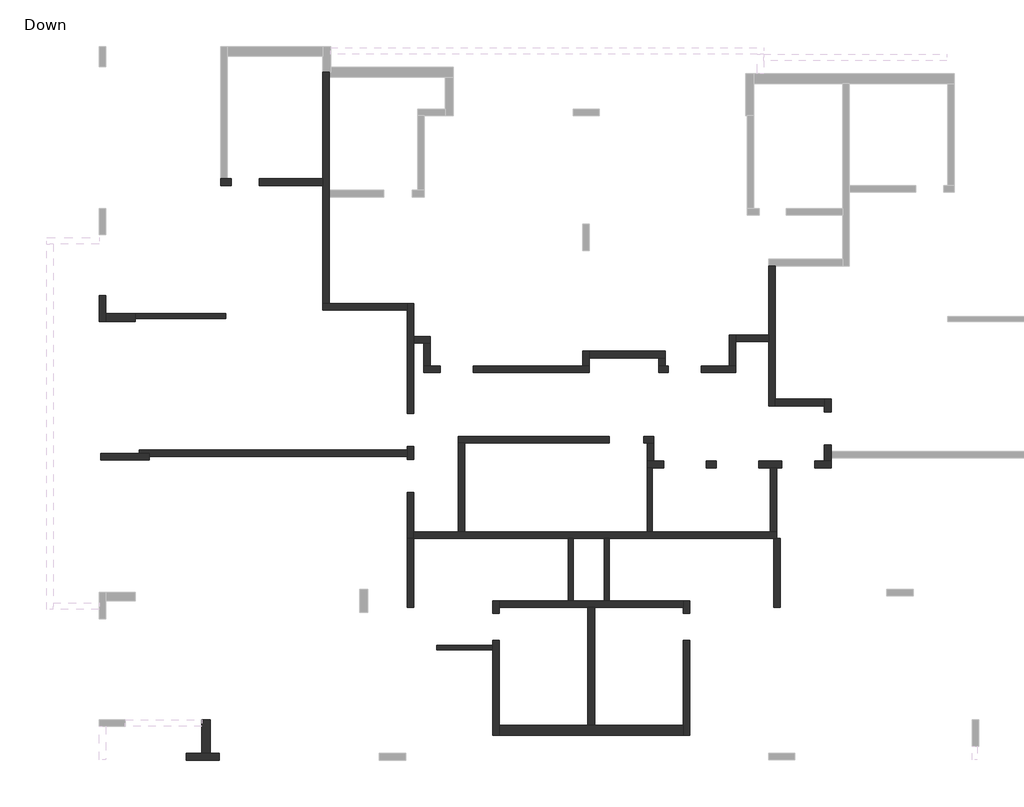
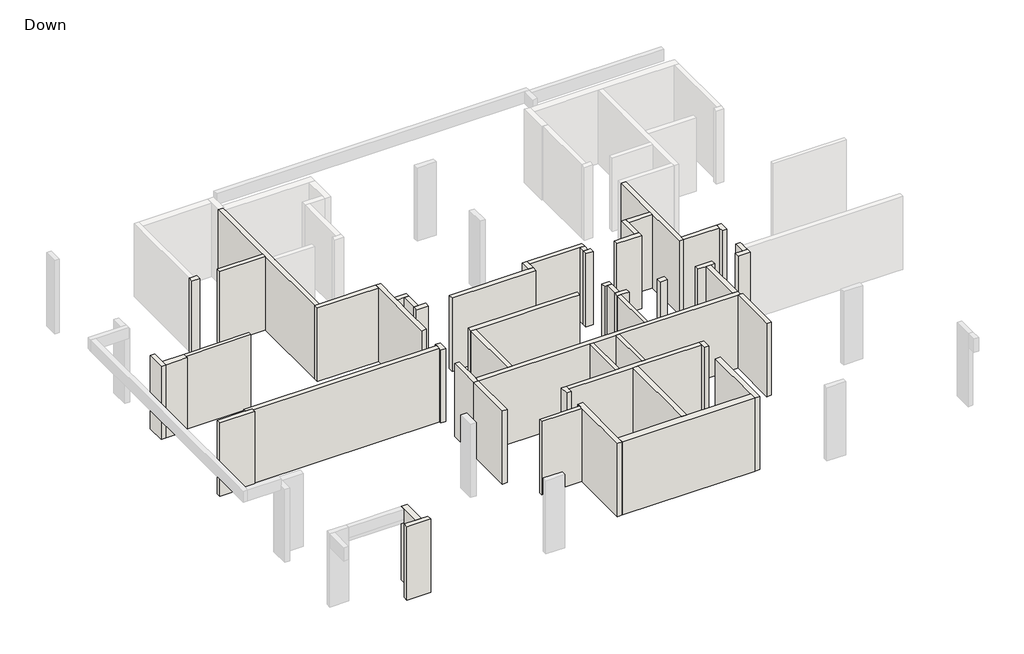
# One storey, part 1 of 2: 52 walls.
"""IFC4 building model written with IfcOpenShell, lengths in millimetres."""

import ifcopenshell
import ifcopenshell.guid

model = None  # the IFC model being written
_history = None  # IfcOwnerHistory: only IFC2X3 demands one
_inside = {}  # id of a spatial element -> (the spatial element, [elements in it])
_under = {}  # id of a project, library or spatial element -> (it, [spatial elements below it])
_declared = {}  # id of a project -> (the project, [libraries it declares])
_typed = {}  # id of a type object -> (the type object, [elements of that type])
_made_of = {}  # id of a material, layer set ... -> (it, [elements and type objects made of it])


def new_model(schema):
    """Start an empty IFC model of exactly this schema.

    Asked for "IFC4X3", IfcOpenShell would pick the latest addendum, in which some entities
    have other attributes; the version numbers below select the first issue.
    IFC2X3 requires an IfcOwnerHistory on every rooted entity: one is made here for all.
    """
    global model, _history
    if schema == "IFC4X3":
        model = ifcopenshell.file(schema_version=(4, 3, 0, 0))
    else:
        model = ifcopenshell.file(schema=schema)
    _inside.clear()
    _under.clear()
    _declared.clear()
    _typed.clear()
    _made_of.clear()
    _history = None
    if model.schema == "IFC2X3":
        org = make("IfcOrganization", Name="unknown")
        user = make(
            "IfcPersonAndOrganization",
            ThePerson=make("IfcPerson", FamilyName="unknown"),
            TheOrganization=org,
        )
        app = make(
            "IfcApplication",
            ApplicationDeveloper=org,
            Version="unknown",
            ApplicationFullName="unknown",
            ApplicationIdentifier="unknown",
        )
        _history = make(
            "IfcOwnerHistory",
            OwningUser=user,
            OwningApplication=app,
            ChangeAction="ADDED",
            CreationDate=0,
        )
    return model


def make(cls, **values):
    """One entity of the class cls with the attributes given. An attribute that is None is left unset."""
    return model.create_entity(
        cls, **{name: value for name, value in values.items() if value is not None}
    )


def rooted(cls, **values):
    """An entity with a GlobalId (a new one), such as an element, a storey or a relation."""
    return make(cls, GlobalId=ifcopenshell.guid.new(), OwnerHistory=_history, **values)


def si_unit(unit_type, name, prefix=None):
    """IfcSIUnit, for example si_unit("LENGTHUNIT", "METRE", prefix="MILLI")."""
    return make("IfcSIUnit", UnitType=unit_type, Prefix=prefix, Name=name)


def assignment(units):
    """IfcUnitAssignment: the units of a project."""
    return None if units is None else make("IfcUnitAssignment", Units=units)


def point(xyz):
    """IfcCartesianPoint."""
    return None if xyz is None else make("IfcCartesianPoint", Coordinates=xyz)


def direction(xyz):
    """IfcDirection."""
    return None if xyz is None else make("IfcDirection", DirectionRatios=xyz)


def frame(location, z_axis=None, x_axis=None):
    """IfcAxis2Placement3D, a coordinate frame: its origin and axes. An axis left out is left unset."""
    return make(
        "IfcAxis2Placement3D",
        Location=point(location),
        Axis=direction(z_axis),
        RefDirection=direction(x_axis),
    )


def origin():
    """The frame at (0, 0, 0) with its axes left unset."""
    return frame((0.0, 0.0, 0.0))


def origin_with_axes():
    """The frame at (0, 0, 0) with the z axis (0, 0, 1) and the x axis (1, 0, 0) written out."""
    return frame((0.0, 0.0, 0.0), z_axis=(0.0, 0.0, 1.0), x_axis=(1.0, 0.0, 0.0))


def place(relative_to, where):
    """IfcLocalPlacement: puts the frame where relative to a parent placement (None: the world)."""
    return make(
        "IfcLocalPlacement", PlacementRelTo=relative_to, RelativePlacement=where
    )


def context(
    kind, dimensions, precision=None, world=None, true_north=None, identifier=None
):
    """IfcGeometricRepresentationContext, for example the 3D "Model" context."""
    return make(
        "IfcGeometricRepresentationContext",
        ContextIdentifier=identifier,
        ContextType=kind,
        CoordinateSpaceDimension=dimensions,
        Precision=precision,
        WorldCoordinateSystem=world,
        TrueNorth=true_north,
    )


def project(units=None, contexts=None):
    """IfcProject with its units and contexts."""
    return rooted(
        "IfcProject",
        Name="project",
        RepresentationContexts=contexts,
        UnitsInContext=assignment(units),
    )


def spatial(cls, under=None, at=None, **own):
    """A site, building, storey or space (cls), placed at a placement, below another one or the project."""
    s = rooted(cls, ObjectPlacement=at, **own)
    if under is not None:
        _under.setdefault(under.id(), (under, []))[1].append(s)
    return s


def polyline(points):
    """IfcPolyline through the points."""
    return make("IfcPolyline", Points=[point(p) for p in points])


def outline(outer, holes=None, kind="AREA"):
    """IfcArbitraryClosedProfileDef: a profile drawn as a closed curve; with holes, ...WithVoids."""
    if holes is None:
        return make("IfcArbitraryClosedProfileDef", ProfileType=kind, OuterCurve=outer)
    return make(
        "IfcArbitraryProfileDefWithVoids",
        ProfileType=kind,
        OuterCurve=outer,
        InnerCurves=holes,
    )


def extrude(swept, where, along, depth):
    """IfcExtrudedAreaSolid: the profile swept, set in the frame where, extruded along a direction by depth."""
    return make(
        "IfcExtrudedAreaSolid",
        SweptArea=swept,
        Position=where,
        ExtrudedDirection=direction(along),
        Depth=depth,
    )


def faces_of(points, faces, orient=None, outer=None):
    """IfcFace entities. A face is a list of loops; a loop is a list of indices into points, from 0.

    orient and outer hold one flag for each loop. By default every Orientation is true, the
    first loop of a face is its IfcFaceOuterBound and the others are IfcFaceBound.
    """
    made = []
    for i, loops in enumerate(faces):
        bounds = []
        for j, loop in enumerate(loops):
            is_outer = j == 0 if outer is None else outer[i][j]
            bounds.append(
                make(
                    "IfcFaceOuterBound" if is_outer else "IfcFaceBound",
                    Bound=make("IfcPolyLoop", Polygon=[points[k] for k in loop]),
                    Orientation=True if orient is None else orient[i][j],
                )
            )
        made.append(make("IfcFace", Bounds=bounds))
    return made


def faceted_brep(points, faces, orient=None, outer=None, voids=None):
    """IfcFacetedBrep: a solid bounded by flat faces; with voids (closed shells), ...WithVoids."""
    shared = [point(p) for p in points]
    hull = make("IfcClosedShell", CfsFaces=faces_of(shared, faces, orient, outer))
    if voids is None:
        return make("IfcFacetedBrep", Outer=hull)
    return make(
        "IfcFacetedBrepWithVoids",
        Outer=hull,
        Voids=[
            make(cls, CfsFaces=faces_of(shared, fs, o, b)) for cls, fs, o, b in voids
        ],
    )


def shape(context_of_items, identifier, shape_type, items):
    """IfcShapeRepresentation: the items that make up one representation, for example the "Body"."""
    return make(
        "IfcShapeRepresentation",
        ContextOfItems=context_of_items,
        RepresentationIdentifier=identifier,
        RepresentationType=shape_type,
        Items=items,
    )


def made_of(thing, what):
    """Note that an element or type object is made of a material, layer set ...; save() writes the relation."""
    if what is not None:
        _made_of.setdefault(what.id(), (what, []))[1].append(thing)
    return thing


def element(
    cls,
    number,
    at=None,
    inside=None,
    cuts=None,
    type_object=None,
    material=None,
    context=None,
    identifier="Body",
    shape_type=None,
    held_by="IfcProductDefinitionShape",
    body=None,
    shapes=None,
    **own,
):
    """One element of the class cls, such as IfcWall. Its Tag is "e" and its number.

    at: its placement. inside: the storey or other place that contains it. cuts: it is an
    opening in that element (IfcRelVoidsElement). A single representation is given by context,
    identifier, shape_type and body (its items); several are given by shapes. held_by: the class
    of the entity that holds the representations. save() writes the other relations.
    """
    e = rooted(cls, Tag="e%d" % number, ObjectPlacement=at, **own)
    if body is not None:
        shapes = [shape(context, identifier, shape_type, body)]
    if shapes is not None:
        e.Representation = make(held_by, Representations=shapes)
    if inside is not None:
        _inside.setdefault(inside.id(), (inside, []))[1].append(e)
    if cuts is not None:
        rooted(
            "IfcRelVoidsElement", RelatingBuildingElement=cuts, RelatedOpeningElement=e
        )
    if type_object is not None:
        _typed.setdefault(type_object.id(), (type_object, []))[1].append(e)
    return made_of(e, material)


def aggregate(whole, parts):
    """IfcRelAggregates: a whole, such as a stair, and the parts it consists of."""
    return rooted("IfcRelAggregates", RelatingObject=whole, RelatedObjects=parts)


def save(model, path):
    """Write the relations noted so far, then the file.

    IfcRelAggregates (storeys below a building ...), IfcRelContainedInSpatialStructure (elements
    in a storey), IfcRelDefinesByType, IfcRelAssociatesMaterial and IfcRelDeclares: one each for
    every whole, place, type object, material and project.
    """
    for whole, parts in _under.values():
        aggregate(whole, parts)
    for where, things in _inside.values():
        rooted(
            "IfcRelContainedInSpatialStructure",
            RelatedElements=things,
            RelatingStructure=where,
        )
    for kind, things in _typed.values():
        rooted("IfcRelDefinesByType", RelatedObjects=things, RelatingType=kind)
    for what, things in _made_of.values():
        rooted("IfcRelAssociatesMaterial", RelatedObjects=things, RelatingMaterial=what)
    for by, libraries in _declared.values():
        rooted("IfcRelDeclares", RelatingContext=by, RelatedDefinitions=libraries)
    model.write(path)


model = new_model("IFC4")

# Units and contexts
model_context = context("Model", 3, world=origin())
ifc_project = project(units=[si_unit("LENGTHUNIT", "METRE", prefix="MILLI")], contexts=[model_context])

# Site, building, storey
site = spatial("IfcSite", under=ifc_project)
building = spatial("IfcBuilding", under=site)
storey = spatial("IfcBuildingStorey", under=building, Name="Down", Elevation=0.0)

# Walls
placement = place(None, origin())
element("IfcWall", 1, ObjectType="15", at=placement, inside=storey, context=model_context, shape_type="Brep", body=[
    faceted_brep([(-7552.8747236, 25916.7313306, 0.0), (-7552.8747236, 23965.2552968, 0.0), (-7552.8747236, 23965.2552968, 3070.0), (-7552.8747236, 23965.2552968, 3270.0), (-7552.8747236, 25916.7313306, 3270.0), (-7402.8747236, 25916.7313306, 0.0), (-7402.8747236, 25916.7313306, 3270.0), (-7402.8747236, 23965.2552968, 3270.0), (-7402.8747236, 23965.2552968, 0.0)], [[[0, 1, 2, 3, 4]], [[5, 6, 7, 8]], [[1, 0, 5, 8]], [[4, 3, 7, 6]], [[0, 4, 6, 5]], [[3, 2, 1, 8, 7]]]),
])
element("IfcWall", 2, ObjectType="15", at=placement, inside=storey, context=model_context, shape_type="Brep", body=[
    faceted_brep([(-8853.5354838, 23765.2552968, 0.0), (-8853.5354838, 21866.6770852, 0.0), (-8853.5354838, 21866.6770852, 3270.0), (-8853.5354838, 23765.2552968, 3270.0), (-8703.5354838, 23765.2552968, 0.0), (-8703.5354838, 23765.2552968, 3070.0), (-8703.5354838, 23765.2552968, 3270.0), (-8703.5354838, 21866.6770852, 3270.0), (-8703.5354838, 21866.6770852, 3070.0), (-8703.5354838, 21866.6770852, 0.0)], [[[0, 1, 2, 3]], [[4, 5, 6, 7, 8, 9]], [[1, 0, 4, 9]], [[3, 2, 7, 6]], [[0, 3, 6, 5, 4]], [[2, 1, 9, 8, 7]]]),
])
element("IfcWall", 3, ObjectType="15", at=placement, inside=storey, context=model_context, shape_type="Brep", body=[
    faceted_brep([(-9801.7338445, 21866.6770852, 0.0), (-9801.7338445, 23765.2552968, 0.0), (-9801.7338445, 23765.2552968, 3270.0), (-9801.7338445, 21866.6770852, 3270.0), (-9951.7338445, 21866.6770852, 0.0), (-9951.7338445, 21866.6770852, 3070.0), (-9951.7338445, 21866.6770852, 3270.0), (-9951.7338445, 23765.2552968, 3270.0), (-9951.7338445, 23765.2552968, 3070.0), (-9951.7338445, 23765.2552968, 0.0)], [[[0, 1, 2, 3]], [[4, 5, 6, 7, 8, 9]], [[1, 0, 4, 9]], [[3, 2, 7, 6]], [[2, 1, 9, 8, 7]], [[0, 3, 6, 5, 4]]]),
])
element("IfcWall", 4, ObjectType="15", at=placement, inside=storey, context=model_context, shape_type="Brep", body=[
    faceted_brep([(-13952.32577, 20366.0504107, 0.0), (-12252.7403699, 20366.0504107, 0.0), (-12252.7403699, 20366.0504107, 3070.0), (-12252.7403699, 20366.0504107, 3270.0), (-13952.32577, 20366.0504107, 3270.0), (-13952.32577, 20366.0504107, 3070.0), (-13952.32577, 20516.0504107, 0.0), (-13952.32577, 20516.0504107, 3070.0), (-13952.32577, 20516.0504107, 3270.0), (-12252.7403699, 20516.0504107, 3270.0), (-12252.7403699, 20516.0504107, 3070.0), (-12252.7403699, 20516.0504107, 0.0)], [[[0, 1, 2, 3, 4, 5]], [[6, 7, 8, 9, 10, 11]], [[1, 0, 6, 11]], [[4, 3, 9, 8]], [[0, 5, 4, 8, 7, 6]], [[3, 2, 1, 11, 10, 9]]]),
])
element("IfcWall", 5, ObjectType="15", at=placement, inside=storey, context=model_context, shape_type="Brep", body=[
    faceted_brep([(-20382.4727235, 30616.5662069, 0.0), (-23131.9002946, 30616.5662069, 0.0), (-23131.9002946, 30616.5662069, 3270.0), (-20382.4727235, 30616.5662069, 3270.0), (-20382.4727235, 30616.5662069, 3070.0), (-20382.4727235, 30466.5662069, 0.0), (-20382.4727235, 30466.5662069, 3070.0), (-20382.4727235, 30466.5662069, 3270.0), (-23131.9002946, 30466.5662069, 3270.0), (-23131.9002946, 30466.5662069, 3070.0), (-23131.9002946, 30466.5662069, 0.0)], [[[0, 1, 2, 3, 4]], [[5, 6, 7, 8, 9, 10]], [[1, 0, 5, 10]], [[2, 1, 10, 9, 8]], [[3, 2, 8, 7]], [[0, 4, 3, 7, 6, 5]]]),
])
element("IfcWall", 6, ObjectType="20", at=placement, inside=storey, context=model_context, shape_type="Brep", body=[
    faceted_brep([(-24181.7083796, 26152.7259194, 0.0), (-22702.2148918, 26152.7259194, 0.0), (-22702.2148918, 26152.7259194, 3070.0), (-22702.2148918, 26152.7259194, 3270.0), (-24181.7083796, 26152.7259194, 3270.0), (-24181.7083796, 26152.7259194, 3070.0), (-24181.7083796, 26352.7259194, 0.0), (-24181.7083796, 26352.7259194, 3070.0), (-24181.7083796, 26352.7259194, 3270.0), (-23002.7833418, 26352.7259194, 3270.0), (-22702.2148918, 26352.7259194, 3270.0), (-22702.2148918, 26352.7259194, 0.0), (-23002.7833418, 26352.7259194, 0.0), (-22702.2148918, 26265.9742814, 0.0), (-22702.2148918, 26265.9742814, 3270.0)], [[[0, 1, 2, 3, 4, 5]], [[6, 7, 8, 9, 10, 11, 12]], [[1, 0, 6, 12, 11, 13]], [[3, 2, 1, 13, 11, 10, 14]], [[4, 3, 14, 10, 9, 8]], [[0, 5, 4, 8, 7, 6]]]),
])
element("IfcWall", 7, ObjectType="20", at=placement, inside=storey, context=model_context, shape_type="Brep", body=[
    faceted_brep([(-14852.9249902, 26265.9742814, 0.0), (-14852.9249902, 26265.9742814, 3070.0), (-14852.9249902, 26265.9742814, 3270.0), (-22702.2148918, 26265.9742814, 3270.0), (-22702.2148918, 26265.9742814, 3070.0), (-22702.2148918, 26265.9742814, 0.0), (-14852.9249902, 26465.9742814, 0.0), (-23002.7833418, 26465.9742814, 0.0), (-23002.7833418, 26465.9742814, 3070.0), (-23002.7833418, 26465.9742814, 3270.0), (-14852.9249902, 26465.9742814, 3270.0), (-14852.9249902, 26465.9742814, 3070.0), (-22702.2148918, 26352.7259194, 0.0), (-23002.7833418, 26352.7259194, 0.0), (-23002.7833418, 26352.7259194, 3270.0), (-22702.2148918, 26352.7259194, 3270.0), (-23002.7833418, 26352.7259194, 3070.0)], [[[0, 1, 2, 3, 4, 5]], [[6, 7, 8, 9, 10, 11]], [[7, 6, 0, 5, 12, 13]], [[10, 9, 14, 15, 3, 2]], [[9, 8, 7, 13, 16, 14]], [[12, 15, 14, 16, 13]], [[15, 12, 5, 4, 3]], [[2, 1, 0, 6, 11, 10]]]),
])
element("IfcWall", 8, ObjectType="20", at=placement, inside=storey, context=model_context, shape_type="Brep", body=[
    faceted_brep([(-14652.9249902, 26165.4399171, 0.0), (-14652.9249902, 26561.209964, 0.0), (-14652.9249902, 26561.209964, 3070.0), (-14652.9249902, 26561.209964, 3270.0), (-14652.9249902, 26165.4399171, 3270.0), (-14652.9249902, 26165.4399171, 3070.0), (-14852.9249902, 26165.4399171, 0.0), (-14852.9249902, 26165.4399171, 3070.0), (-14852.9249902, 26165.4399171, 3270.0), (-14852.9249902, 26265.9742814, 3270.0), (-14852.9249902, 26465.9742814, 3270.0), (-14852.9249902, 26561.209964, 3270.0), (-14852.9249902, 26561.209964, 3070.0), (-14852.9249902, 26561.209964, 0.0), (-14852.9249902, 26465.9742814, 0.0), (-14852.9249902, 26265.9742814, 0.0)], [[[0, 1, 2, 3, 4, 5]], [[6, 7, 8, 9, 10, 11, 12, 13, 14, 15]], [[1, 0, 6, 15, 14, 13]], [[3, 2, 1, 13, 12, 11]], [[4, 3, 11, 10, 9, 8]], [[0, 5, 4, 8, 7, 6]]]),
])
element("IfcWall", 9, ObjectType="20", at=placement, inside=storey, context=model_context, shape_type="Brep", body=[
    faceted_brep([(-14652.9249902, 27566.6042716, 0.0), (-14652.9249902, 29714.8949424, 0.0), (-14652.9249902, 29914.8949424, 0.0), (-14652.9249902, 30914.9872525, 0.0), (-14652.9249902, 30914.9872525, 3070.0), (-14652.9249902, 30914.9872525, 3270.0), (-14652.9249902, 29914.8949424, 3270.0), (-14652.9249902, 29714.8949424, 3270.0), (-14652.9249902, 28915.3710824, 3270.0), (-14652.9249902, 27566.6042716, 3270.0), (-14652.9249902, 27566.6042716, 3070.0), (-14852.9249902, 27566.6042716, 0.0), (-14852.9249902, 27566.6042716, 3070.0), (-14852.9249902, 27566.6042716, 3270.0), (-14852.9249902, 30714.9872525, 3270.0), (-14852.9249902, 30914.9872525, 3270.0), (-14852.9249902, 30914.9872525, 0.0), (-14852.9249902, 30714.9872525, 0.0)], [[[0, 1, 2, 3, 4, 5, 6, 7, 8, 9, 10]], [[11, 12, 13, 14, 15, 16, 17]], [[3, 2, 1, 0, 11, 17, 16]], [[9, 8, 7, 6, 5, 15, 14, 13]], [[0, 10, 9, 13, 12, 11]], [[5, 4, 3, 16, 15]]]),
])
element("IfcWall", 10, ObjectType="20", at=placement, inside=storey, context=model_context, shape_type="Brep", body=[
    faceted_brep([(-14852.9249902, 30914.9872525, 0.0), (-17231.9731082, 30914.9872525, 0.0), (-17431.9731082, 30914.9872525, 0.0), (-17431.9731082, 30914.9872525, 3270.0), (-17231.9731082, 30914.9872525, 3270.0), (-14852.9249902, 30914.9872525, 3270.0), (-14852.9249902, 30714.9872525, 0.0), (-14852.9249902, 30714.9872525, 3070.0), (-14852.9249902, 30714.9872525, 3270.0), (-17431.9731082, 30714.9872525, 3270.0), (-17431.9731082, 30714.9872525, 3070.0), (-17431.9731082, 30714.9872525, 0.0)], [[[0, 1, 2, 3, 4, 5]], [[6, 7, 8, 9, 10, 11]], [[2, 1, 0, 6, 11]], [[5, 4, 3, 9, 8]], [[0, 5, 8, 7, 6]], [[3, 2, 11, 10, 9]]]),
])
element("IfcWall", 11, ObjectType="20", at=placement, inside=storey, context=model_context, shape_type="Brep", body=[
    faceted_brep([(-17231.9731082, 30914.9872525, 0.0), (-17231.9731082, 34166.055318, 0.0), (-17231.9731082, 34366.055318, 0.0), (-17231.9731082, 37815.0067491, 0.0), (-17231.9731082, 37965.0067491, 0.0), (-17231.9731082, 37965.0067491, 3270.0), (-17231.9731082, 37815.0067491, 3270.0), (-17231.9731082, 34366.055318, 3270.0), (-17231.9731082, 34166.055318, 3270.0), (-17231.9731082, 30914.9872525, 3270.0), (-17231.9731082, 30914.9872525, 3070.0), (-17431.9731082, 30914.9872525, 0.0), (-17431.9731082, 30914.9872525, 3270.0), (-17431.9731082, 34515.264183, 3270.0), (-17431.9731082, 34715.264183, 3270.0), (-17431.9731082, 37965.0067491, 3270.0), (-17431.9731082, 37965.0067491, 0.0), (-17431.9731082, 34715.264183, 0.0), (-17431.9731082, 34515.264183, 0.0)], [[[0, 1, 2, 3, 4, 5, 6, 7, 8, 9, 10]], [[11, 12, 13, 14, 15, 16, 17, 18]], [[4, 3, 2, 1, 0, 11, 18, 17, 16]], [[5, 4, 16, 15]], [[9, 8, 7, 6, 5, 15, 14, 13, 12]], [[0, 10, 9, 12, 11]]]),
])
element("IfcWall", 12, ObjectType="20", at=placement, inside=storey, context=model_context, shape_type="Brep", body=[
    faceted_brep([(-20208.9079075, 34715.264183, 0.0), (-20332.7228628, 34715.264183, 0.0), (-20532.7228628, 34715.264183, 0.0), (-20532.7228628, 34715.264183, 3270.0), (-20332.7228628, 34715.264183, 3270.0), (-20208.9079075, 34715.264183, 3270.0), (-20208.9079075, 34715.264183, 3070.0), (-20208.9079075, 34515.264183, 0.0), (-20208.9079075, 34515.264183, 3070.0), (-20208.9079075, 34515.264183, 3270.0), (-20532.7228628, 34515.264183, 3270.0), (-20532.7228628, 34515.264183, 3070.0), (-20532.7228628, 34515.264183, 0.0)], [[[0, 1, 2, 3, 4, 5, 6]], [[7, 8, 9, 10, 11, 12]], [[2, 1, 0, 7, 12]], [[5, 4, 3, 10, 9]], [[0, 6, 5, 9, 8, 7]], [[3, 2, 12, 11, 10]]]),
])
element("IfcWall", 13, ObjectType="20", at=placement, inside=storey, context=model_context, shape_type="Brep", body=[
    faceted_brep([(-19353.797825, 34515.264183, 0.0), (-17431.9731082, 34515.264183, 0.0), (-17431.9731082, 34515.264183, 3070.0), (-17431.9731082, 34515.264183, 3270.0), (-19353.797825, 34515.264183, 3270.0), (-19353.797825, 34515.264183, 3070.0), (-19353.797825, 34715.264183, 0.0), (-19353.797825, 34715.264183, 3070.0), (-19353.797825, 34715.264183, 3270.0), (-17431.9731082, 34715.264183, 3270.0), (-17431.9731082, 34715.264183, 3070.0), (-17431.9731082, 34715.264183, 0.0)], [[[0, 1, 2, 3, 4, 5]], [[6, 7, 8, 9, 10, 11]], [[1, 0, 6, 11]], [[4, 3, 9, 8]], [[0, 5, 4, 8, 7, 6]], [[3, 2, 1, 11, 10, 9]]]),
])
element("IfcWall", 14, ObjectType="20", at=placement, inside=storey, context=model_context, shape_type="Brep", body=[
    faceted_brep([(-14652.9249902, 29714.8949424, 0.0), (-14353.3978144, 29714.8949424, 0.0), (-14153.3978144, 29714.8949424, 0.0), (-14153.3978144, 29714.8949424, 3270.0), (-14353.3978144, 29714.8949424, 3270.0), (-14652.9249902, 29714.8949424, 3270.0), (-14652.9249902, 29914.8949424, 0.0), (-14652.9249902, 29914.8949424, 3070.0), (-14652.9249902, 29914.8949424, 3270.0), (-14153.3978144, 29914.8949424, 3270.0), (-14153.3978144, 29914.8949424, 3070.0), (-14153.3978144, 29914.8949424, 0.0)], [[[0, 1, 2, 3, 4, 5]], [[6, 7, 8, 9, 10, 11]], [[2, 1, 0, 6, 11]], [[5, 4, 3, 9, 8]], [[0, 5, 8, 7, 6]], [[3, 2, 11, 10, 9]]]),
])
element("IfcWall", 15, ObjectType="20", at=placement, inside=storey, context=model_context, shape_type="Brep", body=[
    faceted_brep([(-14353.3978144, 29714.8949424, 0.0), (-14353.3978144, 29015.3710824, 0.0), (-14353.3978144, 29015.3710824, 3270.0), (-14353.3978144, 29714.8949424, 3270.0), (-14153.3978144, 29714.8949424, 0.0), (-14153.3978144, 29714.8949424, 3270.0), (-14153.3978144, 29015.3710824, 3270.0), (-14153.3978144, 29015.3710824, 3070.0), (-14153.3978144, 29015.3710824, 0.0)], [[[0, 1, 2, 3]], [[4, 5, 6, 7, 8]], [[1, 0, 4, 8]], [[3, 2, 6, 5]], [[0, 3, 5, 4]], [[2, 1, 8, 7, 6]]]),
])
element("IfcWall", 16, ObjectType="20", at=placement, inside=storey, context=model_context, shape_type="Brep", body=[
    faceted_brep([(-14353.3978144, 28815.3710824, 0.0), (-13852.8634501, 28815.3710824, 0.0), (-13852.8634501, 28815.3710824, 3070.0), (-13852.8634501, 28815.3710824, 3270.0), (-14353.3978144, 28815.3710824, 3270.0), (-14353.3978144, 28815.3710824, 3070.0), (-14353.3978144, 29015.3710824, 0.0), (-14353.3978144, 29015.3710824, 3270.0), (-14153.3978144, 29015.3710824, 3270.0), (-13852.8634501, 29015.3710824, 3270.0), (-13852.8634501, 29015.3710824, 3070.0), (-13852.8634501, 29015.3710824, 0.0), (-14153.3978144, 29015.3710824, 0.0), (-14353.3978144, 28915.3710824, 3270.0)], [[[0, 1, 2, 3, 4, 5]], [[6, 7, 8, 9, 10, 11, 12]], [[1, 0, 6, 12, 11]], [[3, 2, 1, 11, 10, 9]], [[4, 3, 9, 8, 7, 13]], [[0, 5, 4, 13, 7, 6]]]),
])
element("IfcWall", 17, ObjectType="20", at=placement, inside=storey, context=model_context, shape_type="Brep", body=[
    faceted_brep([(-12851.7298656, 28815.3710824, 0.0), (-9317.0680709, 28815.3710824, 0.0), (-9317.0680709, 28815.3710824, 3070.0), (-9317.0680709, 28815.3710824, 3270.0), (-12851.7298656, 28815.3710824, 3270.0), (-12851.7298656, 28815.3710824, 3070.0), (-12851.7298656, 29015.3710824, 0.0), (-12851.7298656, 29015.3710824, 3070.0), (-12851.7298656, 29015.3710824, 3270.0), (-9517.0680709, 29015.3710824, 3270.0), (-9317.0680709, 29015.3710824, 3270.0), (-9317.0680709, 29015.3710824, 0.0), (-9517.0680709, 29015.3710824, 0.0)], [[[0, 1, 2, 3, 4, 5]], [[6, 7, 8, 9, 10, 11, 12]], [[1, 0, 6, 12, 11]], [[4, 3, 10, 9, 8]], [[0, 5, 4, 8, 7, 6]], [[3, 2, 1, 11, 10]]]),
])
element("IfcWall", 18, ObjectType="20", at=placement, inside=storey, context=model_context, shape_type="Brep", body=[
    faceted_brep([(-9317.0680709, 29015.3710824, 0.0), (-9317.0680709, 29265.1483974, 0.0), (-9317.0680709, 29465.1483974, 0.0), (-9317.0680709, 29465.1483974, 3270.0), (-9317.0680709, 29265.1483974, 3270.0), (-9317.0680709, 29015.3710824, 3270.0), (-9517.0680709, 29015.3710824, 0.0), (-9517.0680709, 29015.3710824, 3070.0), (-9517.0680709, 29015.3710824, 3270.0), (-9517.0680709, 29465.1483974, 3270.0), (-9517.0680709, 29465.1483974, 3070.0), (-9517.0680709, 29465.1483974, 0.0)], [[[0, 1, 2, 3, 4, 5]], [[6, 7, 8, 9, 10, 11]], [[2, 1, 0, 6, 11]], [[5, 4, 3, 9, 8]], [[0, 5, 8, 7, 6]], [[3, 2, 11, 10, 9]]]),
])
element("IfcWall", 19, ObjectType="20", at=placement, inside=storey, context=model_context, shape_type="Brep", body=[
    faceted_brep([(-9317.0680709, 29265.1483974, 0.0), (-7203.6658586, 29265.1483974, 0.0), (-7003.6658586, 29265.1483974, 0.0), (-7003.6658586, 29265.1483974, 3270.0), (-7203.6658586, 29265.1483974, 3270.0), (-9317.0680709, 29265.1483974, 3270.0), (-9317.0680709, 29265.1483974, 3070.0), (-9317.0680709, 29465.1483974, 0.0), (-9317.0680709, 29465.1483974, 3270.0), (-7003.6658586, 29465.1483974, 3270.0), (-7003.6658586, 29465.1483974, 3070.0), (-7003.6658586, 29465.1483974, 0.0)], [[[0, 1, 2, 3, 4, 5, 6]], [[7, 8, 9, 10, 11]], [[2, 1, 0, 7, 11]], [[5, 4, 3, 9, 8]], [[0, 6, 5, 8, 7]], [[3, 2, 11, 10, 9]]]),
])
element("IfcWall", 20, ObjectType="20", at=placement, inside=storey, context=model_context, shape_type="Brep", body=[
    faceted_brep([(-7203.6658586, 29265.1483974, 0.0), (-7203.6658586, 29015.3710824, 0.0), (-7203.6658586, 29015.3710824, 3270.0), (-7203.6658586, 29265.1483974, 3270.0), (-7203.6658586, 29265.1483974, 3070.0), (-7003.6658586, 29265.1483974, 0.0), (-7003.6658586, 29265.1483974, 3270.0), (-7003.6658586, 29015.3710824, 3270.0), (-7003.6658586, 29015.3710824, 3070.0), (-7003.6658586, 29015.3710824, 0.0)], [[[0, 1, 2, 3, 4]], [[5, 6, 7, 8, 9]], [[1, 0, 5, 9]], [[3, 2, 7, 6]], [[0, 4, 3, 6, 5]], [[2, 1, 9, 8, 7]]]),
])
element("IfcWall", 21, ObjectType="20", at=placement, inside=storey, context=model_context, shape_type="Brep", body=[
    faceted_brep([(-7203.6658586, 28815.3710824, 0.0), (-6902.0561342, 28815.3710824, 0.0), (-6902.0561342, 28815.3710824, 3070.0), (-6902.0561342, 28815.3710824, 3270.0), (-7203.6658586, 28815.3710824, 3270.0), (-7203.6658586, 28815.3710824, 3070.0), (-7203.6658586, 29015.3710824, 0.0), (-7203.6658586, 29015.3710824, 3270.0), (-7003.6658586, 29015.3710824, 3270.0), (-6902.0561342, 29015.3710824, 3270.0), (-6902.0561342, 29015.3710824, 3070.0), (-6902.0561342, 29015.3710824, 0.0), (-7003.6658586, 29015.3710824, 0.0)], [[[0, 1, 2, 3, 4, 5]], [[6, 7, 8, 9, 10, 11, 12]], [[1, 0, 6, 12, 11]], [[3, 2, 1, 11, 10, 9]], [[4, 3, 9, 8, 7]], [[0, 5, 4, 7, 6]]]),
])
element("IfcWall", 22, ObjectType="20", at=placement, inside=storey, context=model_context, shape_type="Brep", body=[
    faceted_brep([(-5903.0358684, 28815.3710824, 0.0), (-4853.2277833, 28815.3710824, 0.0), (-4853.2277833, 28815.3710824, 3070.0), (-4853.2277833, 28815.3710824, 3270.0), (-5903.0358684, 28815.3710824, 3270.0), (-5903.0358684, 28815.3710824, 3070.0), (-5903.0358684, 29015.3710824, 0.0), (-5903.0358684, 29015.3710824, 3070.0), (-5903.0358684, 29015.3710824, 3270.0), (-5053.2277833, 29015.3710824, 3270.0), (-4853.2277833, 29015.3710824, 3270.0), (-4853.2277833, 29015.3710824, 0.0), (-5053.2277833, 29015.3710824, 0.0), (-4853.2277833, 28914.6755732, 3270.0)], [[[0, 1, 2, 3, 4, 5]], [[6, 7, 8, 9, 10, 11, 12]], [[1, 0, 6, 12, 11]], [[4, 3, 13, 10, 9, 8]], [[0, 5, 4, 8, 7, 6]], [[3, 2, 1, 11, 10, 13]]]),
])
element("IfcWall", 23, ObjectType="20", at=placement, inside=storey, context=model_context, shape_type="Brep", body=[
    faceted_brep([(-4853.2277833, 29015.3710824, 0.0), (-4853.2277833, 29764.6755732, 0.0), (-4853.2277833, 29964.6755732, 0.0), (-4853.2277833, 29964.6755732, 3270.0), (-4853.2277833, 29764.6755732, 3270.0), (-4853.2277833, 29015.3710824, 3270.0), (-5053.2277833, 29015.3710824, 0.0), (-5053.2277833, 29015.3710824, 3070.0), (-5053.2277833, 29015.3710824, 3270.0), (-5053.2277833, 29964.6755732, 3270.0), (-5053.2277833, 29964.6755732, 3070.0), (-5053.2277833, 29964.6755732, 0.0)], [[[0, 1, 2, 3, 4, 5]], [[6, 7, 8, 9, 10, 11]], [[2, 1, 0, 6, 11]], [[5, 4, 3, 9, 8]], [[0, 5, 8, 7, 6]], [[3, 2, 11, 10, 9]]]),
])
element("IfcWall", 24, ObjectType="20", at=placement, inside=storey, context=model_context, shape_type="Brep", body=[
    faceted_brep([(-4853.2277833, 29764.6755732, 0.0), (-3852.0941989, 29764.6755732, 0.0), (-3852.0941989, 29764.6755732, 3270.0), (-4853.2277833, 29764.6755732, 3270.0), (-4853.2277833, 29964.6755732, 0.0), (-4853.2277833, 29964.6755732, 3270.0), (-3852.0941989, 29964.6755732, 3270.0), (-3852.0941989, 29964.6755732, 3070.0), (-3852.0941989, 29964.6755732, 0.0)], [[[0, 1, 2, 3]], [[4, 5, 6, 7, 8]], [[1, 0, 4, 8]], [[3, 2, 6, 5]], [[0, 3, 5, 4]], [[2, 1, 8, 7, 6]]]),
])
element("IfcWall", 25, ObjectType="20", at=placement, inside=storey, context=model_context, shape_type="Brep", body=[
    faceted_brep([(-8703.2512588, 26864.9330071, 0.0), (-13303.2512588, 26864.9330071, 0.0), (-13303.2512588, 26864.9330071, 3070.0), (-13303.2512588, 26864.9330071, 3270.0), (-8703.2512588, 26864.9330071, 3270.0), (-8703.2512588, 26864.9330071, 3070.0), (-8703.2512588, 26664.9330071, 0.0), (-8703.2512588, 26664.9330071, 3070.0), (-8703.2512588, 26664.9330071, 3270.0), (-9003.2512588, 26664.9330071, 3270.0), (-13102.548455, 26664.9330071, 3270.0), (-13302.548455, 26664.9330071, 3270.0), (-13303.2512588, 26664.9330071, 3270.0), (-13303.2512588, 26664.9330071, 3070.0), (-13303.2512588, 26664.9330071, 0.0), (-13302.548455, 26664.9330071, 0.0), (-13102.548455, 26664.9330071, 0.0)], [[[0, 1, 2, 3, 4, 5]], [[6, 7, 8, 9, 10, 11, 12, 13, 14, 15, 16]], [[1, 0, 6, 16, 15, 14]], [[3, 2, 1, 14, 13, 12]], [[4, 3, 12, 11, 10, 9, 8]], [[0, 5, 4, 8, 7, 6]]]),
])
element("IfcWall", 26, ObjectType="20", at=placement, inside=storey, context=model_context, shape_type="Brep", body=[
    faceted_brep([(-13302.548455, 26664.9330071, 0.0), (-13302.548455, 23965.2552968, 0.0), (-13302.548455, 23965.2552968, 3070.0), (-13302.548455, 23965.2552968, 3270.0), (-13302.548455, 26664.9330071, 3270.0), (-13302.548455, 26664.9330071, 3070.0), (-13102.548455, 26664.9330071, 0.0), (-13102.548455, 26664.9330071, 3270.0), (-13102.548455, 23965.2552968, 3270.0), (-13102.548455, 23965.2552968, 0.0)], [[[0, 1, 2, 3, 4, 5]], [[6, 7, 8, 9]], [[1, 0, 6, 9]], [[4, 3, 8, 7]], [[0, 5, 4, 7, 6]], [[3, 2, 1, 9, 8]]]),
])
element("IfcWall", 27, ObjectType="20", at=placement, inside=storey, context=model_context, shape_type="Brep", body=[
    faceted_brep([(-14851.8837159, 25164.3063326, 0.0), (-14851.8837159, 23765.2552968, 0.0), (-14851.8837159, 23765.2552968, 3270.0), (-14851.8837159, 25164.3063326, 3270.0), (-14851.8837159, 25164.3063326, 3070.0), (-14651.8837159, 25164.3063326, 0.0), (-14651.8837159, 25164.3063326, 3070.0), (-14651.8837159, 25164.3063326, 3270.0), (-14651.8837159, 23965.2552968, 3270.0), (-14651.8837159, 23765.2552968, 3270.0), (-14651.8837159, 23765.2552968, 0.0), (-14651.8837159, 23965.2552968, 0.0), (-14652.9249902, 25164.3063326, 3270.0)], [[[0, 1, 2, 3, 4]], [[5, 6, 7, 8, 9, 10, 11]], [[1, 0, 5, 11, 10]], [[3, 2, 9, 8, 7, 12]], [[0, 4, 3, 12, 7, 6, 5]], [[2, 1, 10, 9]]]),
])
element("IfcWall", 28, ObjectType="20", at=placement, inside=storey, context=model_context, shape_type="Brep", body=[
    faceted_brep([(-14651.8837159, 23765.2552968, 0.0), (-9951.7338445, 23765.2552968, 0.0), (-9801.7338445, 23765.2552968, 0.0), (-8853.5354838, 23765.2552968, 0.0), (-8703.5354838, 23765.2552968, 0.0), (-3702.8512482, 23765.2552968, 0.0), (-3602.3135681, 23765.2552968, 0.0), (-3602.3135681, 23765.2552968, 3070.0), (-3602.3135681, 23765.2552968, 3270.0), (-3702.8512482, 23765.2552968, 3270.0), (-8703.5354838, 23765.2552968, 3270.0), (-8853.5354838, 23765.2552968, 3270.0), (-9801.7338445, 23765.2552968, 3270.0), (-9951.7338445, 23765.2552968, 3270.0), (-14651.8837159, 23765.2552968, 3270.0), (-14651.8837159, 23765.2552968, 3070.0), (-14651.8837159, 23965.2552968, 0.0), (-14651.8837159, 23965.2552968, 3070.0), (-14651.8837159, 23965.2552968, 3270.0), (-13302.548455, 23965.2552968, 3270.0), (-13102.548455, 23965.2552968, 3270.0), (-9538.2512588, 23965.2552968, 3270.0), (-7552.8747236, 23965.2552968, 3270.0), (-7402.8747236, 23965.2552968, 3270.0), (-3802.3135681, 23965.2552968, 3270.0), (-3602.3135681, 23965.2552968, 3270.0), (-3602.3135681, 23965.2552968, 0.0), (-3802.3135681, 23965.2552968, 0.0), (-7402.8747236, 23965.2552968, 0.0), (-7552.8747236, 23965.2552968, 0.0), (-13102.548455, 23965.2552968, 0.0), (-13302.548455, 23965.2552968, 0.0)], [[[0, 1, 2, 3, 4, 5, 6, 7, 8, 9, 10, 11, 12, 13, 14, 15]], [[16, 17, 18, 19, 20, 21, 22, 23, 24, 25, 26, 27, 28, 29, 30, 31]], [[6, 5, 4, 3, 2, 1, 0, 16, 31, 30, 29, 28, 27, 26]], [[14, 13, 12, 11, 10, 9, 8, 25, 24, 23, 22, 21, 20, 19, 18]], [[0, 15, 14, 18, 17, 16]], [[8, 7, 6, 26, 25]]]),
])
element("IfcWall", 29, ObjectType="20", at=placement, inside=storey, context=model_context, shape_type="Brep", body=[
    faceted_brep([(-3602.3135681, 23965.2552968, 0.0), (-3602.3135681, 25916.7313306, 0.0), (-3602.3135681, 25916.7313306, 3070.0), (-3602.3135681, 25916.7313306, 3270.0), (-3602.3135681, 23965.2552968, 3270.0), (-3802.3135681, 23965.2552968, 0.0), (-3802.3135681, 23965.2552968, 3270.0), (-3802.3135681, 25916.7313306, 3270.0), (-3802.3135681, 25916.7313306, 0.0)], [[[0, 1, 2, 3, 4]], [[5, 6, 7, 8]], [[1, 0, 5, 8]], [[4, 3, 7, 6]], [[0, 4, 6, 5]], [[3, 2, 1, 8, 7]]]),
])
element("IfcWall", 30, ObjectType="20", at=placement, inside=storey, context=model_context, shape_type="Brep", body=[
    faceted_brep([(-3452.0634289, 26116.7313306, 0.0), (-4152.6285632, 26116.7313306, 0.0), (-4152.6285632, 26116.7313306, 3270.0), (-3452.0634289, 26116.7313306, 3270.0), (-3452.0634289, 26116.7313306, 3070.0), (-3452.0634289, 25916.7313306, 0.0), (-3452.0634289, 25916.7313306, 3070.0), (-3452.0634289, 25916.7313306, 3270.0), (-3602.3135681, 25916.7313306, 3270.0), (-3802.3135681, 25916.7313306, 3270.0), (-4152.6285632, 25916.7313306, 3270.0), (-4152.6285632, 25916.7313306, 0.0), (-3802.3135681, 25916.7313306, 0.0), (-3602.3135681, 25916.7313306, 0.0)], [[[0, 1, 2, 3, 4]], [[5, 6, 7, 8, 9, 10, 11, 12, 13]], [[1, 0, 5, 13, 12, 11]], [[2, 1, 11, 10]], [[3, 2, 10, 9, 8, 7]], [[0, 4, 3, 7, 6, 5]]]),
])
element("IfcWall", 31, ObjectType="20", at=placement, inside=storey, context=model_context, shape_type="SweptSolid", body=[
    extrude(outline(polyline([(-5750.6383247, 26116.7313306), (-5452.2172791, 26116.7313306), (-5452.2172791, 25916.7313306), (-5750.6383247, 25916.7313306), (-5750.6383247, 26116.7313306)])), origin_with_axes(), (0.0, 0.0, 1.0), 3270.0),
])
element("IfcWall", 32, ObjectType="20", at=placement, inside=storey, context=model_context, shape_type="Brep", body=[
    faceted_brep([(-7052.3403593, 26116.7313306, 0.0), (-7352.8747236, 26116.7313306, 0.0), (-7552.8747236, 26116.7313306, 0.0), (-7552.8747236, 26116.7313306, 3270.0), (-7352.8747236, 26116.7313306, 3270.0), (-7052.3403593, 26116.7313306, 3270.0), (-7052.3403593, 25916.7313306, 0.0), (-7052.3403593, 25916.7313306, 3270.0), (-7402.8747236, 25916.7313306, 3270.0), (-7552.8747236, 25916.7313306, 3270.0), (-7552.8747236, 25916.7313306, 0.0), (-7402.8747236, 25916.7313306, 0.0)], [[[0, 1, 2, 3, 4, 5]], [[6, 7, 8, 9, 10, 11]], [[2, 1, 0, 6, 11, 10]], [[5, 4, 3, 9, 8, 7]], [[0, 5, 7, 6]], [[3, 2, 10, 9]]]),
])
element("IfcWall", 33, ObjectType="20", at=placement, inside=storey, context=model_context, shape_type="Brep", body=[
    faceted_brep([(-7653.4431737, 26666.0050514, 0.0), (-7552.8747236, 26666.0050514, 0.0), (-7352.8747236, 26666.0050514, 0.0), (-7352.8747236, 26666.0050514, 3270.0), (-7552.8747236, 26666.0050514, 3270.0), (-7653.4431737, 26666.0050514, 3270.0), (-7653.4431737, 26666.0050514, 3070.0), (-7653.4431737, 26866.0050514, 0.0), (-7653.4431737, 26866.0050514, 3070.0), (-7653.4431737, 26866.0050514, 3270.0), (-7352.8747236, 26866.0050514, 3270.0), (-7352.8747236, 26866.0050514, 3070.0), (-7352.8747236, 26866.0050514, 0.0)], [[[0, 1, 2, 3, 4, 5, 6]], [[7, 8, 9, 10, 11, 12]], [[2, 1, 0, 7, 12]], [[5, 4, 3, 10, 9]], [[0, 6, 5, 9, 8, 7]], [[3, 2, 12, 11, 10]]]),
])
element("IfcWall", 34, ObjectType="20", at=placement, inside=storey, context=model_context, shape_type="Brep", body=[
    faceted_brep([(-7552.8747236, 26666.0050514, 0.0), (-7552.8747236, 26116.7313306, 0.0), (-7552.8747236, 26116.7313306, 3270.0), (-7552.8747236, 26666.0050514, 3270.0), (-7552.8747236, 26666.0050514, 3070.0), (-7352.8747236, 26666.0050514, 0.0), (-7352.8747236, 26666.0050514, 3270.0), (-7352.8747236, 26116.7313306, 3270.0), (-7352.8747236, 26116.7313306, 3070.0), (-7352.8747236, 26116.7313306, 0.0)], [[[0, 1, 2, 3, 4]], [[5, 6, 7, 8, 9]], [[1, 0, 5, 9]], [[3, 2, 7, 6]], [[2, 1, 9, 8, 7]], [[0, 4, 3, 6, 5]]]),
])
element("IfcWall", 35, ObjectType="20", at=placement, inside=storey, context=model_context, shape_type="Brep", body=[
    faceted_brep([(-3502.8512482, 21665.6050408, 0.0), (-3502.8512482, 23765.2552968, 0.0), (-3502.8512482, 23765.2552968, 3070.0), (-3502.8512482, 23765.2552968, 3270.0), (-3502.8512482, 21665.6050408, 3270.0), (-3502.8512482, 21665.6050408, 3070.0), (-3702.8512482, 21665.6050408, 0.0), (-3702.8512482, 21665.6050408, 3070.0), (-3702.8512482, 21665.6050408, 3270.0), (-3702.8512482, 23765.2552968, 3270.0), (-3702.8512482, 23765.2552968, 3070.0), (-3702.8512482, 23765.2552968, 0.0), (-3602.3135681, 23765.2552968, 0.0), (-3602.3135681, 23765.2552968, 3270.0)], [[[0, 1, 2, 3, 4, 5]], [[6, 7, 8, 9, 10, 11]], [[1, 0, 6, 11, 12]], [[4, 3, 13, 9, 8]], [[0, 5, 4, 8, 7, 6]], [[3, 2, 1, 12, 11, 10, 9, 13]]]),
])
element("IfcWall", 36, ObjectType="20", at=placement, inside=storey, context=model_context, shape_type="Brep", body=[
    faceted_brep([(-12052.7403699, 17775.3603394, 0.0), (-12052.7403699, 18075.3603394, 0.0), (-12052.7403699, 20656.0181817, 0.0), (-12052.7403699, 20656.0181817, 3070.0), (-12052.7403699, 20656.0181817, 3270.0), (-12052.7403699, 18075.3603394, 3270.0), (-12052.7403699, 17775.3603394, 3270.0), (-12252.7403699, 17775.3603394, 0.0), (-12252.7403699, 17775.3603394, 3070.0), (-12252.7403699, 17775.3603394, 3270.0), (-12252.7403699, 20366.0504107, 3270.0), (-12252.7403699, 20516.0504107, 3270.0), (-12252.7403699, 20656.0181817, 3270.0), (-12252.7403699, 20656.0181817, 0.0), (-12252.7403699, 20516.0504107, 0.0), (-12252.7403699, 20366.0504107, 0.0)], [[[0, 1, 2, 3, 4, 5, 6]], [[7, 8, 9, 10, 11, 12, 13, 14, 15]], [[2, 1, 0, 7, 15, 14, 13]], [[4, 3, 2, 13, 12]], [[6, 5, 4, 12, 11, 10, 9]], [[0, 6, 9, 8, 7]]]),
])
element("IfcWall", 37, ObjectType="20", at=placement, inside=storey, context=model_context, shape_type="Brep", body=[
    faceted_brep([(-12052.7403699, 21476.6770852, 0.0), (-12052.7403699, 21666.6770852, 0.0), (-12052.7403699, 21866.6770852, 0.0), (-12052.7403699, 21866.6770852, 3270.0), (-12052.7403699, 21666.6770852, 3270.0), (-12052.7403699, 21476.6770852, 3270.0), (-12052.7403699, 21476.6770852, 3070.0), (-12252.7403699, 21476.6770852, 0.0), (-12252.7403699, 21476.6770852, 3270.0), (-12252.7403699, 21866.6770852, 3270.0), (-12252.7403699, 21866.6770852, 3070.0), (-12252.7403699, 21866.6770852, 0.0)], [[[0, 1, 2, 3, 4, 5, 6]], [[7, 8, 9, 10, 11]], [[2, 1, 0, 7, 11]], [[5, 4, 3, 9, 8]], [[0, 6, 5, 8, 7]], [[3, 2, 11, 10, 9]]]),
])
element("IfcWall", 38, ObjectType="20", at=placement, inside=storey, context=model_context, shape_type="Brep", body=[
    faceted_brep([(-12052.7403699, 21666.6770852, 0.0), (-9353.0285738, 21666.6770852, 0.0), (-9153.0285738, 21666.6770852, 0.0), (-6453.3508635, 21666.6770852, 0.0), (-6453.3508635, 21666.6770852, 3070.0), (-6453.3508635, 21666.6770852, 3270.0), (-9153.0285738, 21666.6770852, 3270.0), (-9353.0285738, 21666.6770852, 3270.0), (-12052.7403699, 21666.6770852, 3270.0), (-12052.7403699, 21866.6770852, 0.0), (-12052.7403699, 21866.6770852, 3270.0), (-9951.7338445, 21866.6770852, 3270.0), (-9801.7338445, 21866.6770852, 3270.0), (-8853.5354838, 21866.6770852, 3270.0), (-8703.5354838, 21866.6770852, 3270.0), (-6453.3508635, 21866.6770852, 3270.0), (-6453.3508635, 21866.6770852, 0.0), (-8703.5354838, 21866.6770852, 0.0), (-8853.5354838, 21866.6770852, 0.0), (-9801.7338445, 21866.6770852, 0.0), (-9951.7338445, 21866.6770852, 0.0)], [[[0, 1, 2, 3, 4, 5, 6, 7, 8]], [[9, 10, 11, 12, 13, 14, 15, 16, 17, 18, 19, 20]], [[3, 2, 1, 0, 9, 20, 19, 18, 17, 16]], [[8, 7, 6, 5, 15, 14, 13, 12, 11, 10]], [[0, 8, 10, 9]], [[5, 4, 3, 16, 15]]]),
])
element("IfcWall", 39, ObjectType="20", at=placement, inside=storey, context=model_context, shape_type="Brep", body=[
    faceted_brep([(-6453.3508635, 21866.6770852, 0.0), (-6453.3508635, 21666.6770852, 0.0), (-6453.3508635, 21476.6770852, 0.0), (-6453.3508635, 21476.6770852, 3070.0), (-6453.3508635, 21476.6770852, 3270.0), (-6453.3508635, 21666.6770852, 3270.0), (-6453.3508635, 21866.6770852, 3270.0), (-6253.3508635, 21866.6770852, 0.0), (-6253.3508635, 21866.6770852, 3070.0), (-6253.3508635, 21866.6770852, 3270.0), (-6253.3508635, 21476.6770852, 3270.0), (-6253.3508635, 21476.6770852, 3070.0), (-6253.3508635, 21476.6770852, 0.0)], [[[0, 1, 2, 3, 4, 5, 6]], [[7, 8, 9, 10, 11, 12]], [[2, 1, 0, 7, 12]], [[4, 3, 2, 12, 11, 10]], [[6, 5, 4, 10, 9]], [[0, 6, 9, 8, 7]]]),
])
element("IfcWall", 40, ObjectType="20", at=placement, inside=storey, context=model_context, shape_type="Brep", body=[
    faceted_brep([(-9353.0285738, 21666.6770852, 0.0), (-9353.0285738, 18075.3603394, 0.0), (-9353.0285738, 18075.3603394, 3070.0), (-9353.0285738, 18075.3603394, 3270.0), (-9353.0285738, 21666.6770852, 3270.0), (-9353.0285738, 21666.6770852, 3070.0), (-9153.0285738, 21666.6770852, 0.0), (-9153.0285738, 21666.6770852, 3070.0), (-9153.0285738, 21666.6770852, 3270.0), (-9153.0285738, 18075.3603394, 3270.0), (-9153.0285738, 18075.3603394, 3070.0), (-9153.0285738, 18075.3603394, 0.0)], [[[0, 1, 2, 3, 4, 5]], [[6, 7, 8, 9, 10, 11]], [[1, 0, 6, 11]], [[4, 3, 9, 8]], [[3, 2, 1, 11, 10, 9]], [[0, 5, 4, 8, 7, 6]]]),
])
element("IfcWall", 41, ObjectType="20", at=placement, inside=storey, context=model_context, shape_type="Brep", body=[
    faceted_brep([(-14651.8837159, 21665.6050408, 0.0), (-14651.8837159, 23765.2552968, 0.0), (-14651.8837159, 23765.2552968, 3070.0), (-14651.8837159, 23765.2552968, 3270.0), (-14651.8837159, 21665.6050408, 3270.0), (-14651.8837159, 21665.6050408, 3070.0), (-14851.8837159, 21665.6050408, 0.0), (-14851.8837159, 21665.6050408, 3070.0), (-14851.8837159, 21665.6050408, 3270.0), (-14851.8837159, 23765.2552968, 3270.0), (-14851.8837159, 23765.2552968, 0.0)], [[[0, 1, 2, 3, 4, 5]], [[6, 7, 8, 9, 10]], [[1, 0, 6, 10]], [[4, 3, 9, 8]], [[0, 5, 4, 8, 7, 6]], [[3, 2, 1, 10, 9]]]),
])
element("IfcWall", 42, ObjectType="20", at=placement, inside=storey, context=model_context, shape_type="Brep", body=[
    faceted_brep([(-6453.3508635, 20656.0181817, 0.0), (-6453.3508635, 18075.3603394, 0.0), (-6453.3508635, 17775.3603394, 0.0), (-6453.3508635, 17775.3603394, 3270.0), (-6453.3508635, 18075.3603394, 3270.0), (-6453.3508635, 20656.0181817, 3270.0), (-6453.3508635, 20656.0181817, 3070.0), (-6253.3508635, 20656.0181817, 0.0), (-6253.3508635, 20656.0181817, 3070.0), (-6253.3508635, 20656.0181817, 3270.0), (-6253.3508635, 17775.3603394, 3270.0), (-6253.3508635, 17775.3603394, 3070.0), (-6253.3508635, 17775.3603394, 0.0), (-6452.0326588, 17775.3603394, 3270.0)], [[[0, 1, 2, 3, 4, 5, 6]], [[7, 8, 9, 10, 11, 12]], [[2, 1, 0, 7, 12]], [[5, 4, 3, 13, 10, 9]], [[0, 6, 5, 9, 8, 7]], [[3, 2, 12, 11, 10, 13]]]),
])
element("IfcWall", 43, ObjectType="20", at=placement, inside=storey, context=model_context, shape_type="Brep", body=[
    faceted_brep([(-3852.0941989, 32066.405062, 0.0), (-3852.0941989, 29964.6755732, 0.0), (-3852.0941989, 29764.6755732, 0.0), (-3852.0941989, 27804.6755732, 0.0), (-3852.0941989, 27804.6755732, 3070.0), (-3852.0941989, 27804.6755732, 3270.0), (-3852.0941989, 28914.6755732, 3270.0), (-3852.0941989, 29764.6755732, 3270.0), (-3852.0941989, 29964.6755732, 3270.0), (-3852.0941989, 32066.405062, 3270.0), (-3652.0941989, 32066.405062, 0.0), (-3652.0941989, 32066.405062, 3070.0), (-3652.0941989, 32066.405062, 3270.0), (-3652.0941989, 28004.6755732, 3270.0), (-3652.0941989, 27804.6755732, 3270.0), (-3652.0941989, 27804.6755732, 0.0), (-3652.0941989, 28004.6755732, 0.0)], [[[0, 1, 2, 3, 4, 5, 6, 7, 8, 9]], [[10, 11, 12, 13, 14, 15, 16]], [[3, 2, 1, 0, 10, 16, 15]], [[9, 8, 7, 6, 5, 14, 13, 12]], [[0, 9, 12, 11, 10]], [[5, 4, 3, 15, 14]]]),
])
element("IfcWall", 44, ObjectType="20", at=placement, inside=storey, context=model_context, shape_type="Brep", body=[
    faceted_brep([(-3652.0941989, 27804.6755732, 0.0), (-2153.6864162, 27804.6755732, 0.0), (-2153.6864162, 27804.6755732, 3070.0), (-2153.6864162, 27804.6755732, 3270.0), (-3652.0941989, 27804.6755732, 3270.0), (-3652.0941989, 28004.6755732, 0.0), (-3652.0941989, 28004.6755732, 3070.0), (-3652.0941989, 28004.6755732, 3270.0), (-2153.6864162, 28004.6755732, 3270.0), (-2153.6864162, 28004.6755732, 0.0)], [[[0, 1, 2, 3, 4]], [[5, 6, 7, 8, 9]], [[1, 0, 5, 9]], [[4, 3, 8, 7]], [[0, 4, 7, 6, 5]], [[3, 2, 1, 9, 8]]]),
])
element("IfcWall", 45, ObjectType="20", at=placement, inside=storey, context=model_context, shape_type="Brep", body=[
    faceted_brep([(-2153.6864162, 28004.6755732, 0.0), (-2153.6864162, 27804.6755732, 0.0), (-2153.6864162, 27615.2787722, 0.0), (-2153.6864162, 27615.2787722, 3070.0), (-2153.6864162, 27615.2787722, 3270.0), (-2153.6864162, 27804.6755732, 3270.0), (-2153.6864162, 28004.6755732, 3270.0), (-1953.6864162, 28004.6755732, 0.0), (-1953.6864162, 28004.6755732, 3070.0), (-1953.6864162, 28004.6755732, 3270.0), (-1953.6864162, 27615.2787722, 3270.0), (-1953.6864162, 27615.2787722, 3070.0), (-1953.6864162, 27615.2787722, 0.0)], [[[0, 1, 2, 3, 4, 5, 6]], [[7, 8, 9, 10, 11, 12]], [[2, 1, 0, 7, 12]], [[4, 3, 2, 12, 11, 10]], [[6, 5, 4, 10, 9]], [[0, 6, 9, 8, 7]]]),
])
element("IfcWall", 46, ObjectType="20", at=placement, inside=storey, context=model_context, shape_type="Brep", body=[
    faceted_brep([(-2453.0431631, 25916.7313306, 0.0), (-1953.6864162, 25916.7313306, 0.0), (-1953.6864162, 25916.7313306, 3070.0), (-1953.6864162, 25916.7313306, 3270.0), (-2453.0431631, 25916.7313306, 3270.0), (-2453.0431631, 25916.7313306, 3070.0), (-2453.0431631, 26116.7313306, 0.0), (-2453.0431631, 26116.7313306, 3070.0), (-2453.0431631, 26116.7313306, 3270.0), (-2153.6864162, 26116.7313306, 3270.0), (-1953.6864162, 26116.7313306, 3270.0), (-1953.6864162, 26116.7313306, 0.0), (-2153.6864162, 26116.7313306, 0.0)], [[[0, 1, 2, 3, 4, 5]], [[6, 7, 8, 9, 10, 11, 12]], [[1, 0, 6, 12, 11]], [[4, 3, 10, 9, 8]], [[0, 5, 4, 8, 7, 6]], [[3, 2, 1, 11, 10]]]),
])
element("IfcWall", 47, ObjectType="20", at=placement, inside=storey, context=model_context, shape_type="Brep", body=[
    faceted_brep([(-1953.6864162, 26116.7313306, 0.0), (-1953.6864162, 26215.1864621, 0.0), (-1953.6864162, 26415.1864621, 0.0), (-1953.6864162, 26616.2585064, 0.0), (-1953.6864162, 26616.2585064, 3070.0), (-1953.6864162, 26616.2585064, 3270.0), (-1953.6864162, 26415.1864621, 3270.0), (-1953.6864162, 26215.1864621, 3270.0), (-1953.6864162, 26116.7313306, 3270.0), (-2153.6864162, 26116.7313306, 0.0), (-2153.6864162, 26116.7313306, 3070.0), (-2153.6864162, 26116.7313306, 3270.0), (-2153.6864162, 26616.2585064, 3270.0), (-2153.6864162, 26616.2585064, 3070.0), (-2153.6864162, 26616.2585064, 0.0)], [[[0, 1, 2, 3, 4, 5, 6, 7, 8]], [[9, 10, 11, 12, 13, 14]], [[3, 2, 1, 0, 9, 14]], [[5, 4, 3, 14, 13, 12]], [[8, 7, 6, 5, 12, 11]], [[0, 8, 11, 10, 9]]]),
])
element("IfcWall", 48, ObjectType="20", at=placement, inside=storey, context=model_context, shape_type="Brep", body=[
    faceted_brep([(-24032.496199, 30366.5662069, 0.0), (-24032.496199, 30616.5662069, 0.0), (-24032.496199, 31164.7337975, 0.0), (-24032.496199, 31164.7337975, 3070.0), (-24032.496199, 31164.7337975, 3270.0), (-24032.496199, 30616.5662069, 3270.0), (-24032.496199, 30366.5662069, 3270.0), (-24232.496199, 30366.5662069, 0.0), (-24232.496199, 30366.5662069, 3070.0), (-24232.496199, 30366.5662069, 3270.0), (-24232.496199, 31164.7337975, 3270.0), (-24232.496199, 31164.7337975, 3070.0), (-24232.496199, 31164.7337975, 0.0)], [[[0, 1, 2, 3, 4, 5, 6]], [[7, 8, 9, 10, 11, 12]], [[2, 1, 0, 7, 12]], [[4, 3, 2, 12, 11, 10]], [[6, 5, 4, 10, 9]], [[0, 6, 9, 8, 7]]]),
])
element("IfcWall", 49, ObjectType="20", at=placement, inside=storey, context=model_context, shape_type="Brep", body=[
    faceted_brep([(-20572.9440888, 17215.5200253, 0.0), (-20852.3452666, 17215.5200253, 0.0), (-21102.3452666, 17215.5200253, 0.0), (-21571.9643546, 17215.5200253, 0.0), (-21571.9643546, 17215.5200253, 2670.0), (-21571.9643546, 17215.5200253, 2820.0), (-21571.9643546, 17215.5200253, 3270.0), (-21102.3452666, 17215.5200253, 3270.0), (-20852.3452666, 17215.5200253, 3270.0), (-20572.9440888, 17215.5200253, 3270.0), (-20572.9440888, 17215.5200253, 3070.0), (-20572.9440888, 17015.5200253, 0.0), (-20572.9440888, 17015.5200253, 3070.0), (-20572.9440888, 17015.5200253, 3270.0), (-21571.9643546, 17015.5200253, 3270.0), (-21571.9643546, 17015.5200253, 0.0)], [[[0, 1, 2, 3, 4, 5, 6, 7, 8, 9, 10]], [[11, 12, 13, 14, 15]], [[3, 2, 1, 0, 11, 15]], [[6, 5, 4, 3, 15, 14]], [[9, 8, 7, 6, 14, 13]], [[0, 10, 9, 13, 12, 11]]]),
])
element("IfcWall", 50, ObjectType="25", at=placement, inside=storey, context=model_context, shape_type="Brep", body=[
    faceted_brep([(-23131.9002946, 30616.5662069, 0.0), (-24032.496199, 30616.5662069, 0.0), (-24032.496199, 30616.5662069, 3070.0), (-24032.496199, 30616.5662069, 3270.0), (-23131.9002946, 30616.5662069, 3270.0), (-23131.9002946, 30366.5662069, 0.0), (-23131.9002946, 30366.5662069, 3070.0), (-23131.9002946, 30366.5662069, 3270.0), (-24032.496199, 30366.5662069, 3270.0), (-24032.496199, 30366.5662069, 0.0), (-23131.9002946, 30466.5662069, 0.0), (-23131.9002946, 30466.5662069, 3270.0)], [[[0, 1, 2, 3, 4]], [[5, 6, 7, 8, 9]], [[1, 0, 10, 5, 9]], [[4, 3, 8, 7, 11]], [[0, 4, 11, 7, 6, 5, 10]], [[3, 2, 1, 9, 8]]]),
])
element("IfcWall", 51, ObjectType="25", at=placement, inside=storey, context=model_context, shape_type="Brep", body=[
    faceted_brep([(-21102.3452666, 18236.7796078, 0.0), (-21102.3452666, 17215.5200253, 0.0), (-21102.3452666, 17215.5200253, 2670.0), (-21102.3452666, 17215.5200253, 2820.0), (-21102.3452666, 17215.5200253, 3270.0), (-21102.3452666, 18236.7796078, 3270.0), (-20852.3452666, 18236.7796078, 0.0), (-20852.3452666, 18236.7796078, 3070.0), (-20852.3452666, 18236.7796078, 3270.0), (-20852.3452666, 17215.5200253, 3270.0), (-20852.3452666, 17215.5200253, 3070.0), (-20852.3452666, 17215.5200253, 0.0)], [[[0, 1, 2, 3, 4, 5]], [[6, 7, 8, 9, 10, 11]], [[1, 0, 6, 11]], [[5, 4, 9, 8]], [[0, 5, 8, 7, 6]], [[4, 3, 2, 1, 11, 10, 9]]]),
])
element("IfcWall", 52, ObjectType="30", at=placement, inside=storey, context=model_context, shape_type="Brep", body=[
    faceted_brep([(-6453.3508635, 18075.3603394, 0.0), (-9153.0285738, 18075.3603394, 0.0), (-9353.0285738, 18075.3603394, 0.0), (-12052.7403699, 18075.3603394, 0.0), (-12052.7403699, 18075.3603394, 3270.0), (-9353.0285738, 18075.3603394, 3270.0), (-9153.0285738, 18075.3603394, 3270.0), (-6453.3508635, 18075.3603394, 3270.0), (-6453.3508635, 18075.3603394, 3070.0), (-6453.3508635, 17775.3603394, 0.0), (-6453.3508635, 17775.3603394, 3270.0), (-12051.6683255, 17775.3603394, 3270.0), (-12052.7403699, 17775.3603394, 3270.0), (-12052.7403699, 17775.3603394, 0.0)], [[[0, 1, 2, 3, 4, 5, 6, 7, 8]], [[9, 10, 11, 12, 13]], [[3, 2, 1, 0, 9, 13]], [[7, 6, 5, 4, 12, 11, 10]], [[0, 8, 7, 10, 9]], [[4, 3, 13, 12]]]),
])

save(model, "model.ifc")

# Revit data of these elements
# Project information
#   Project Issue Date = "Issue Date"
#   Project Status = "Project Status"
#   Client Name = "לקוח"
#   Project Address = "Enter address here"
#   Project Name = "Project 011"
#   Project Number = "מספר פרויקט"
# Type "15"
#   Layers, outside or top first: 15 cm "Concrete" (function 1)
# Type "20"
#   Layers, outside or top first: 20 cm "Concrete" (function 1)
# Type "25"
#   Layers, outside or top first: 25 cm "Concrete" (function 1)
# Type "30"
#   Layers, outside or top first: 30 cm "Concrete" (function 1)
# Element 1 (IfcWall, "15")
#   Comments = ""
#   Mark = "W70"
#   SOFiSTiK_EdgeZones = "W72"
#   SOFiSTiK_AMG_Comments = ""
#   Top Offset = 0 cm
#   Base Offset = 0 cm
#   wall height = 327 cm
#   SOFiSTiK_AMG_Scheduled = yes
#   SOFiSTiK_AMG_Adjusted = yes
#   Phase Created = New Construction
#   Base Constraint = Down
#   Top Constraint = Typical Floor
#   Materials on its faces: "Concrete"
# Element 2 (IfcWall, "15")
#   Comments = ""
#   Mark = "W71"
#   SOFiSTiK_EdgeZones = "W73"
#   SOFiSTiK_AMG_Comments = ""
#   Top Offset = 0 cm
#   Base Offset = 0 cm
#   wall height = 327 cm
#   SOFiSTiK_AMG_Scheduled = yes
#   SOFiSTiK_AMG_Adjusted = yes
#   Phase Created = New Construction
#   Base Constraint = Down
#   Top Constraint = Typical Floor
#   Materials on its faces: "Concrete"
# Element 3 (IfcWall, "15")
#   Comments = ""
#   Mark = "W72"
#   SOFiSTiK_EdgeZones = "W74"
#   SOFiSTiK_AMG_Comments = ""
#   Top Offset = 0 cm
#   Base Offset = 0 cm
#   wall height = 327 cm
#   SOFiSTiK_AMG_Scheduled = yes
#   SOFiSTiK_AMG_Adjusted = yes
#   Phase Created = New Construction
#   Base Constraint = Down
#   Top Constraint = Typical Floor
#   Materials on its faces: "Concrete"
